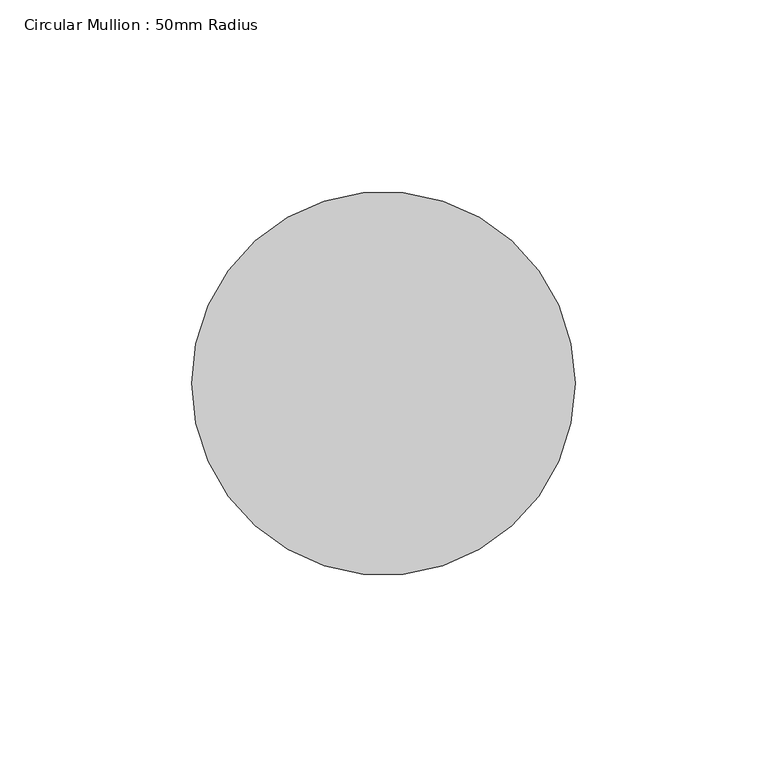
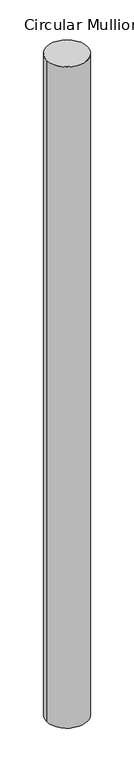
"""IFC4 building model written with IfcOpenShell, lengths in millimetres: member geometry, Circular Mullion : 50mm Radius."""

from ifc_helpers import new_model, si_unit, point, frame, origin, origin_2d, place, context, project, spatial, circle_curve, trimmed, segment, composite_curve, outline, extrude, source, transform, mapped, element, save


def circular_mullion_50mm_radius_45e76bfc(model_context):
    return source(origin(), model_context, "Body", "SweptSolid", [
        extrude(outline(composite_curve([segment(trimmed(circle_curve(origin_2d(), 50.0), [point((50.0, 0.0))], [point((-50.0, 0.0))], False, "CARTESIAN"), True, "CONTINUOUS"), segment(trimmed(circle_curve(origin_2d(), 50.0), [point((-50.0, 0.0))], [point((50.0, 0.0))], False, "CARTESIAN"), True, "CONTINUOUS")], self_intersect=False)), frame((0.0, 0.0, -1706.1354403), z_axis=(0.0, 0.0, 1.0), x_axis=(1.0, 0.0, 0.0)), (0.0, 0.0, 1.0), 1706.1354403),
    ])


if __name__ == "__main__":
    model = new_model("IFC4")
    model_context = context("Model", 3, world=origin())
    ifc_project = project(units=[si_unit("LENGTHUNIT", "METRE", prefix="MILLI")], contexts=[model_context])
    site = spatial("IfcSite", under=ifc_project)
    building = spatial("IfcBuilding", under=site)
    placement = place(None, origin())
    circular_mullion_50mm_radius_shape = circular_mullion_50mm_radius_45e76bfc(model_context)
    element("IfcMember", 1, ObjectType="Circular Mullion : 50mm Radius", at=placement, inside=building, context=model_context, shape_type="MappedRepresentation", body=[
        mapped(circular_mullion_50mm_radius_shape, transform((0.0, 0.0, 0.0), x_axis=(1.0, 0.0, 0.0), y_axis=(0.0, 1.0, 0.0), z_axis=(0.0, 0.0, 1.0))),
    ])
    save(model, "model.ifc")

# Revit data of these elements
# Type "Circular Mullion : 50mm Radius"
#   built-in parameter 1007350 = 0.164042 (stored number, unit not read)
# Element 1 (IfcMember, "Circular Mullion : 50mm Radius")
#   Materials on its faces: "Aluminium"
# Materials
#   "Aluminium": class "Metal", colour RGB 247 247 247, transparency 0, Description = "Aluminium 6061", Cost = 0
